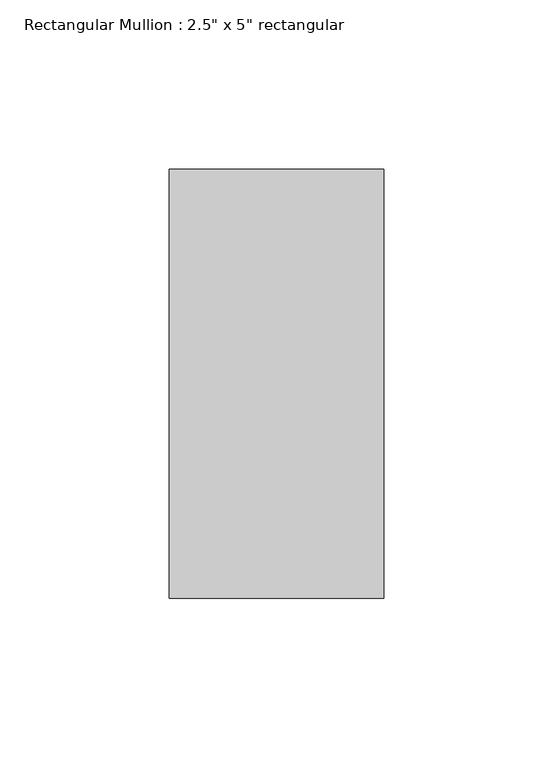
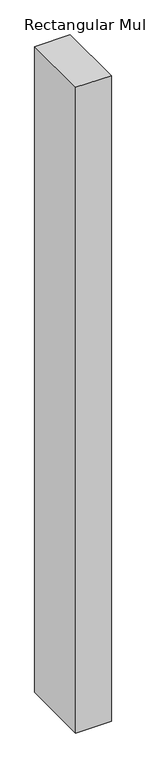
"""IFC4 building model written with IfcOpenShell, lengths in millimetres: member geometry."""

import ifcopenshell
import ifcopenshell.guid

model = None  # the IFC model being written
_history = None  # IfcOwnerHistory: only IFC2X3 demands one
_inside = {}  # id of a spatial element -> (the spatial element, [elements in it])
_under = {}  # id of a project, library or spatial element -> (it, [spatial elements below it])
_declared = {}  # id of a project -> (the project, [libraries it declares])
_typed = {}  # id of a type object -> (the type object, [elements of that type])
_made_of = {}  # id of a material, layer set ... -> (it, [elements and type objects made of it])


def new_model(schema):
    """Start an empty IFC model of exactly this schema.

    Asked for "IFC4X3", IfcOpenShell would pick the latest addendum, in which some entities
    have other attributes; the version numbers below select the first issue.
    IFC2X3 requires an IfcOwnerHistory on every rooted entity: one is made here for all.
    """
    global model, _history
    if schema == "IFC4X3":
        model = ifcopenshell.file(schema_version=(4, 3, 0, 0))
    else:
        model = ifcopenshell.file(schema=schema)
    _inside.clear()
    _under.clear()
    _declared.clear()
    _typed.clear()
    _made_of.clear()
    _history = None
    if model.schema == "IFC2X3":
        org = make("IfcOrganization", Name="unknown")
        user = make(
            "IfcPersonAndOrganization",
            ThePerson=make("IfcPerson", FamilyName="unknown"),
            TheOrganization=org,
        )
        app = make(
            "IfcApplication",
            ApplicationDeveloper=org,
            Version="unknown",
            ApplicationFullName="unknown",
            ApplicationIdentifier="unknown",
        )
        _history = make(
            "IfcOwnerHistory",
            OwningUser=user,
            OwningApplication=app,
            ChangeAction="ADDED",
            CreationDate=0,
        )
    return model


def make(cls, **values):
    """One entity of the class cls with the attributes given. An attribute that is None is left unset."""
    return model.create_entity(
        cls, **{name: value for name, value in values.items() if value is not None}
    )


def rooted(cls, **values):
    """An entity with a GlobalId (a new one), such as an element, a storey or a relation."""
    return make(cls, GlobalId=ifcopenshell.guid.new(), OwnerHistory=_history, **values)


def si_unit(unit_type, name, prefix=None):
    """IfcSIUnit, for example si_unit("LENGTHUNIT", "METRE", prefix="MILLI")."""
    return make("IfcSIUnit", UnitType=unit_type, Prefix=prefix, Name=name)


def assignment(units):
    """IfcUnitAssignment: the units of a project."""
    return None if units is None else make("IfcUnitAssignment", Units=units)


def point(xyz):
    """IfcCartesianPoint."""
    return None if xyz is None else make("IfcCartesianPoint", Coordinates=xyz)


def direction(xyz):
    """IfcDirection."""
    return None if xyz is None else make("IfcDirection", DirectionRatios=xyz)


def frame(location, z_axis=None, x_axis=None):
    """IfcAxis2Placement3D, a coordinate frame: its origin and axes. An axis left out is left unset."""
    return make(
        "IfcAxis2Placement3D",
        Location=point(location),
        Axis=direction(z_axis),
        RefDirection=direction(x_axis),
    )


def origin():
    """The frame at (0, 0, 0) with its axes left unset."""
    return frame((0.0, 0.0, 0.0))


def place(relative_to, where):
    """IfcLocalPlacement: puts the frame where relative to a parent placement (None: the world)."""
    return make(
        "IfcLocalPlacement", PlacementRelTo=relative_to, RelativePlacement=where
    )


def context(
    kind, dimensions, precision=None, world=None, true_north=None, identifier=None
):
    """IfcGeometricRepresentationContext, for example the 3D "Model" context."""
    return make(
        "IfcGeometricRepresentationContext",
        ContextIdentifier=identifier,
        ContextType=kind,
        CoordinateSpaceDimension=dimensions,
        Precision=precision,
        WorldCoordinateSystem=world,
        TrueNorth=true_north,
    )


def project(units=None, contexts=None):
    """IfcProject with its units and contexts."""
    return rooted(
        "IfcProject",
        Name="project",
        RepresentationContexts=contexts,
        UnitsInContext=assignment(units),
    )


def spatial(cls, under=None, at=None, **own):
    """A site, building, storey or space (cls), placed at a placement, below another one or the project."""
    s = rooted(cls, ObjectPlacement=at, **own)
    if under is not None:
        _under.setdefault(under.id(), (under, []))[1].append(s)
    return s


def polyline(points):
    """IfcPolyline through the points."""
    return make("IfcPolyline", Points=[point(p) for p in points])


def outline(outer, holes=None, kind="AREA"):
    """IfcArbitraryClosedProfileDef: a profile drawn as a closed curve; with holes, ...WithVoids."""
    if holes is None:
        return make("IfcArbitraryClosedProfileDef", ProfileType=kind, OuterCurve=outer)
    return make(
        "IfcArbitraryProfileDefWithVoids",
        ProfileType=kind,
        OuterCurve=outer,
        InnerCurves=holes,
    )


def extrude(swept, where, along, depth):
    """IfcExtrudedAreaSolid: the profile swept, set in the frame where, extruded along a direction by depth."""
    return make(
        "IfcExtrudedAreaSolid",
        SweptArea=swept,
        Position=where,
        ExtrudedDirection=direction(along),
        Depth=depth,
    )


def shape(context_of_items, identifier, shape_type, items):
    """IfcShapeRepresentation: the items that make up one representation, for example the "Body"."""
    return make(
        "IfcShapeRepresentation",
        ContextOfItems=context_of_items,
        RepresentationIdentifier=identifier,
        RepresentationType=shape_type,
        Items=items,
    )


def source(mapping_origin, context_of_items, identifier, shape_type, items):
    """IfcRepresentationMap: a shape defined once, which mapped items show again and again."""
    return make(
        "IfcRepresentationMap",
        MappingOrigin=mapping_origin,
        MappedRepresentation=shape(context_of_items, identifier, shape_type, items),
    )


def transform(
    local_origin,
    x_axis=None,
    y_axis=None,
    z_axis=None,
    scale=None,
    scale2=None,
    scale3=None,
    uniform=True,
):
    """IfcCartesianTransformationOperator3D, or its non-uniform kind. x_axis, y_axis, z_axis: its Axis1, 2, 3."""
    if uniform:
        return make(
            "IfcCartesianTransformationOperator3D",
            Axis1=direction(x_axis),
            Axis2=direction(y_axis),
            LocalOrigin=point(local_origin),
            Scale=scale,
            Axis3=direction(z_axis),
        )
    return make(
        "IfcCartesianTransformationOperator3DnonUniform",
        Axis1=direction(x_axis),
        Axis2=direction(y_axis),
        LocalOrigin=point(local_origin),
        Scale=scale,
        Axis3=direction(z_axis),
        Scale2=scale2,
        Scale3=scale3,
    )


def mapped(mapping_source, mapping_target):
    """IfcMappedItem: shows the shape of a source again, moved by a transform."""
    return make(
        "IfcMappedItem", MappingSource=mapping_source, MappingTarget=mapping_target
    )


def made_of(thing, what):
    """Note that an element or type object is made of a material, layer set ...; save() writes the relation."""
    if what is not None:
        _made_of.setdefault(what.id(), (what, []))[1].append(thing)
    return thing


def element(
    cls,
    number,
    at=None,
    inside=None,
    cuts=None,
    type_object=None,
    material=None,
    context=None,
    identifier="Body",
    shape_type=None,
    held_by="IfcProductDefinitionShape",
    body=None,
    shapes=None,
    **own,
):
    """One element of the class cls, such as IfcWall. Its Tag is "e" and its number.

    at: its placement. inside: the storey or other place that contains it. cuts: it is an
    opening in that element (IfcRelVoidsElement). A single representation is given by context,
    identifier, shape_type and body (its items); several are given by shapes. held_by: the class
    of the entity that holds the representations. save() writes the other relations.
    """
    e = rooted(cls, Tag="e%d" % number, ObjectPlacement=at, **own)
    if body is not None:
        shapes = [shape(context, identifier, shape_type, body)]
    if shapes is not None:
        e.Representation = make(held_by, Representations=shapes)
    if inside is not None:
        _inside.setdefault(inside.id(), (inside, []))[1].append(e)
    if cuts is not None:
        rooted(
            "IfcRelVoidsElement", RelatingBuildingElement=cuts, RelatedOpeningElement=e
        )
    if type_object is not None:
        _typed.setdefault(type_object.id(), (type_object, []))[1].append(e)
    return made_of(e, material)


def aggregate(whole, parts):
    """IfcRelAggregates: a whole, such as a stair, and the parts it consists of."""
    return rooted("IfcRelAggregates", RelatingObject=whole, RelatedObjects=parts)


def save(model, path):
    """Write the relations noted so far, then the file.

    IfcRelAggregates (storeys below a building ...), IfcRelContainedInSpatialStructure (elements
    in a storey), IfcRelDefinesByType, IfcRelAssociatesMaterial and IfcRelDeclares: one each for
    every whole, place, type object, material and project.
    """
    for whole, parts in _under.values():
        aggregate(whole, parts)
    for where, things in _inside.values():
        rooted(
            "IfcRelContainedInSpatialStructure",
            RelatedElements=things,
            RelatingStructure=where,
        )
    for kind, things in _typed.values():
        rooted("IfcRelDefinesByType", RelatedObjects=things, RelatingType=kind)
    for what, things in _made_of.values():
        rooted("IfcRelAssociatesMaterial", RelatedObjects=things, RelatingMaterial=what)
    for by, libraries in _declared.values():
        rooted("IfcRelDeclares", RelatingContext=by, RelatedDefinitions=libraries)
    model.write(path)


def member_75074519(model_context):
    return source(origin(), model_context, "Body", "SweptSolid", [
        extrude(outline(polyline([(0.0, 63.5), (0.0, -63.5), (-63.5, -63.5), (-63.5, 63.5), (0.0, 63.5)])), frame((0.0, 0.0, -1219.2), z_axis=(0.0, 0.0, 1.0), x_axis=(1.0, 0.0, 0.0)), (0.0, 0.0, 1.0), 1219.2),
    ])


if __name__ == "__main__":
    model = new_model("IFC4")
    model_context = context("Model", 3, world=origin())
    ifc_project = project(units=[si_unit("LENGTHUNIT", "METRE", prefix="MILLI")], contexts=[model_context])
    site = spatial("IfcSite", under=ifc_project)
    building = spatial("IfcBuilding", under=site)
    placement = place(None, origin())
    member_shape = member_75074519(model_context)
    element("IfcMember", 1, ObjectType="Rectangular Mullion : 2.5\" x 5\" rectangular", at=placement, inside=building, context=model_context, shape_type="MappedRepresentation", body=[
        mapped(member_shape, transform((0.0, 0.0, 0.0), x_axis=(1.0, 0.0, 0.0), y_axis=(0.0, 1.0, 0.0), z_axis=(0.0, 0.0, 1.0))),
    ])
    save(model, "model.ifc")

# Revit data of these elements
# Type "Rectangular Mullion : 2.5\" x 5\" rectangular"
#   built-in parameter 1007304 = 0.416667 (stored number, unit not read)
#   built-in parameter 1007301 = 0.104167 (stored number, unit not read)
#   built-in parameter 1007300 = 0.104167 (stored number, unit not read)
# Element 1 (IfcMember, "Rectangular Mullion : 2.5\" x 5\" rectangular")
#   Materials on its faces: "Aluminum"
# Materials
#   "Aluminum": class "Metal", colour RGB 247 247 247, transparency 0, Description = "Aluminum 6061", Cost = 0
